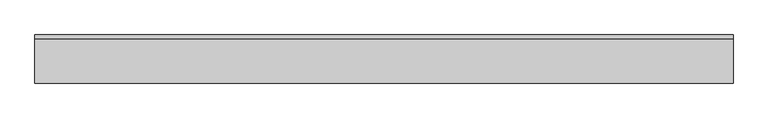
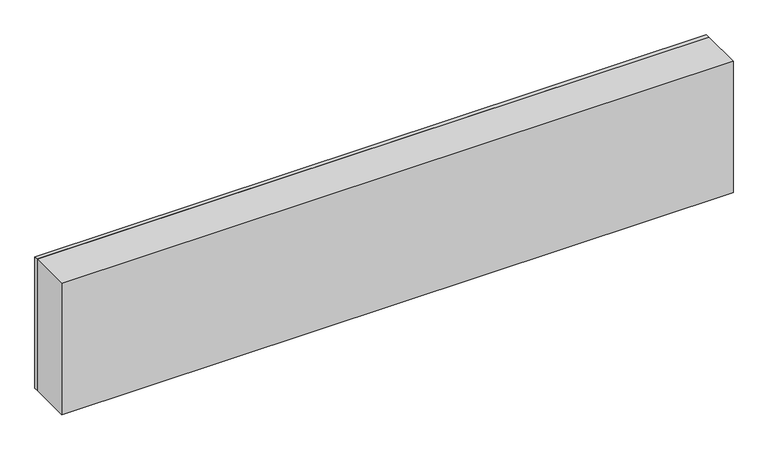
"""IFC4 building model written with IfcOpenShell, lengths in millimetres: furniture geometry, OD_CW_Upper Cabinet : OD_CW_Upper Cabinet."""

from ifc_helpers import new_model, si_unit, frame, origin, place, context, project, spatial, polyline, outline, extrude, source, transform, mapped, element, save


def furniture_746d2c86(model_context):
    return source(origin(), model_context, "Body", "SweptSolid", [
        extrude(outline(polyline([(18.7377049, -330.2), (18.7377049, -304.8), (4438.3377049, -304.8), (4438.3377049, -330.2), (18.7377049, -330.2)])), frame((0.0, 0.0, 965.2), z_axis=(0.0, 0.0, 1.0), x_axis=(1.0, 0.0, 0.0)), (0.0, 0.0, 1.0), 914.4),
        extrude(outline(polyline([(18.7377049, -609.6), (18.7377049, -330.2), (4438.3377049, -330.2), (4438.3377049, -609.6), (18.7377049, -609.6)])), frame((0.0, 0.0, 965.2), z_axis=(0.0, 0.0, 1.0), x_axis=(1.0, 0.0, 0.0)), (0.0, 0.0, 1.0), 914.4),
    ])


if __name__ == "__main__":
    model = new_model("IFC4")
    model_context = context("Model", 3, world=origin())
    ifc_project = project(units=[si_unit("LENGTHUNIT", "METRE", prefix="MILLI")], contexts=[model_context])
    site = spatial("IfcSite", under=ifc_project)
    building = spatial("IfcBuilding", under=site)
    placement = place(None, origin())
    furniture_shape = furniture_746d2c86(model_context)
    element("IfcFurniture", 1, ObjectType="OD_CW_Upper Cabinet : OD_CW_Upper Cabinet", at=placement, inside=building, context=model_context, shape_type="MappedRepresentation", body=[
        mapped(furniture_shape, transform((0.0, 0.0, 0.0), x_axis=(1.0, 0.0, 0.0), y_axis=(0.0, 1.0, 0.0), z_axis=(0.0, 0.0, 1.0))),
    ])
    save(model, "model.ifc")

# Revit data of these elements
# Type "OD_CW_Upper Cabinet : OD_CW_Upper Cabinet"
#   OD_CW_Width [instance default] = 2' - 2"
#   OD_CW_Off Floor [instance default] = 3' - 2"
#   OD_CW_Length [instance default] = 8' - 0"
#   OD_CW_Height [instance default] = 7' - 0"
#   Depth = 2' - 0"
#   Height = 3' - 0"
#   Width = 4' - 0"
#   OD_CW_Material_Front Panel [instance default] = none
# Element 1 (IfcFurniture, "OD_CW_Upper Cabinet : OD_CW_Upper Cabinet")
#   OD_CW_Width = 1' - 0"
#   OD_CW_Length = 14' - 6"
#   OD_CW_Height = 3' - 0"
#   Materials on its faces: "CASEWORK"
# Materials
#   "CASEWORK": class "Generic", colour RGB 181 181 181, transparency 0, Cost = 0
